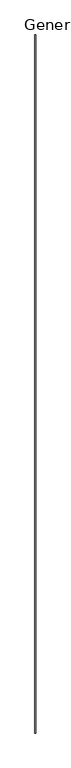
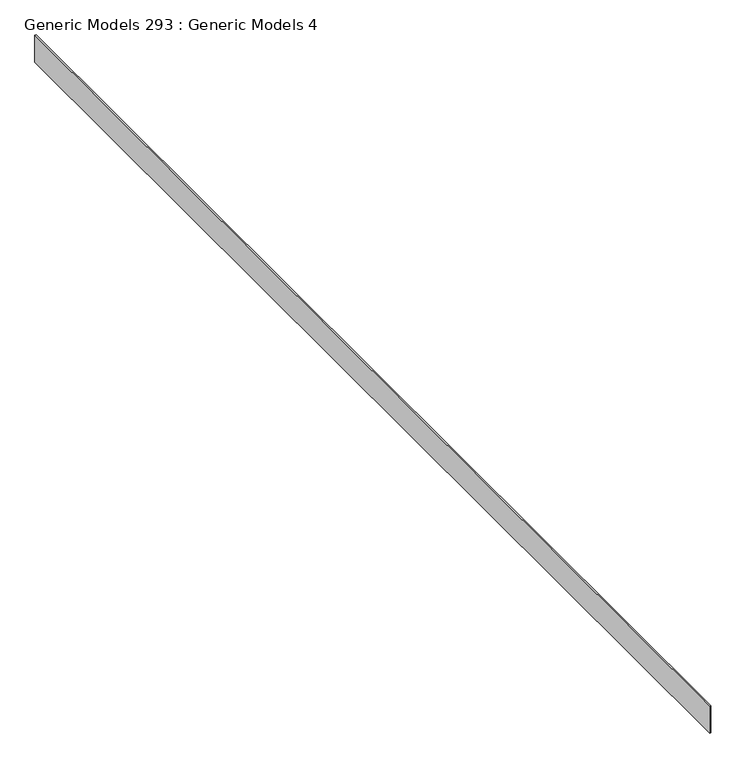
"""IFC4 building model written with IfcOpenShell, lengths in millimetres: proxy geometry, Generic Models 293 : Generic Models 4."""

from ifc_helpers import new_model, si_unit, frame, origin, place, context, project, spatial, polyline, outline, extrude, source, transform, mapped, element, save


def generic_models_293_generic_models_4_05e6c145(model_context):
    return source(origin(), model_context, "Body", "SweptSolid", [
        extrude(outline(polyline([(26420.1627812, 26848.7591064), (26401.1127812, 26848.7591064), (26401.1127812, 45492.3591064), (26420.1627812, 45492.3591064), (26420.1627812, 26848.7591064)])), frame((0.0, 0.0, 125818.8444117), z_axis=(0.0, 0.0, 1.0), x_axis=(1.0, 0.0, 0.0)), (0.0, 0.0, 1.0), 455.4843275),
    ])


if __name__ == "__main__":
    model = new_model("IFC4")
    model_context = context("Model", 3, world=origin())
    ifc_project = project(units=[si_unit("LENGTHUNIT", "METRE", prefix="MILLI")], contexts=[model_context])
    site = spatial("IfcSite", under=ifc_project)
    building = spatial("IfcBuilding", under=site)
    placement = place(None, origin())
    generic_models_293_generic_models_4_shape = generic_models_293_generic_models_4_05e6c145(model_context)
    element("IfcBuildingElementProxy", 1, Name="Generic Models 293 : Generic Models 4", ObjectType="Generic Models 293 : Generic Models 4", at=placement, inside=building, context=model_context, shape_type="MappedRepresentation", body=[
        mapped(generic_models_293_generic_models_4_shape, transform((0.0, 0.0, 0.0), x_axis=(1.0, 0.0, 0.0), y_axis=(0.0, 1.0, 0.0), z_axis=(0.0, 0.0, 1.0))),
    ])
    save(model, "model.ifc")

# Revit data of these elements
# Element 1 (IfcBuildingElementProxy, "Generic Models 293 : Generic Models 4")
#   Materials on its faces: "_CDX PLYWOOD - SEE STRUCT DWGs"
# Materials
#   "_CDX PLYWOOD - SEE STRUCT DWGs": class "Generic", colour RGB 98 75 74, transparency 0, Cost = 0
